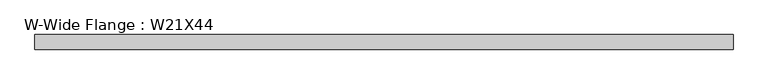
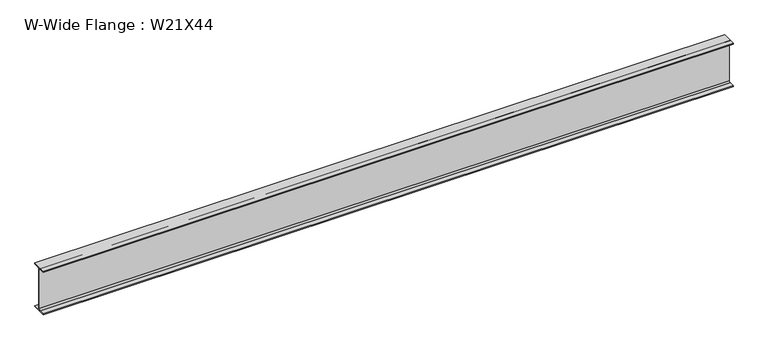
"""IFC4 building model written with IfcOpenShell, lengths in millimetres: beam geometry, W-Wide Flange : W21X44."""

from ifc_helpers import new_model, si_unit, point, frame, frame_2d, origin, place, context, project, spatial, polyline, circle_curve, trimmed, segment, composite_curve, outline, extrude, source, transform, mapped, element, save


def w_wide_flange_w21x44_a0252540(model_context):
    return source(origin(), model_context, "Body", "SweptSolid", [
        extrude(outline(composite_curve([segment(polyline([(82.55, -251.46), (82.55, -262.89), (-82.55, -262.89), (-82.55, -251.46), (-21.59, -251.46)]), True, "CONTINUOUS"), segment(trimmed(circle_curve(frame_2d((-21.59, -234.315)), 17.145), [point((-21.59, -251.46))], [point((-4.445, -234.315))], True, "CARTESIAN"), True, "CONTINUOUS"), segment(polyline([(-4.445, -234.315), (-4.445, 234.315)]), True, "CONTINUOUS"), segment(trimmed(circle_curve(frame_2d((-21.59, 234.315)), 17.145), [point((-4.445, 234.315))], [point((-21.59, 251.46))], True, "CARTESIAN"), True, "CONTINUOUS"), segment(polyline([(-21.59, 251.46), (-82.55, 251.46), (-82.55, 262.89), (82.55, 262.89), (82.55, 251.46), (21.59, 251.46)]), True, "CONTINUOUS"), segment(trimmed(circle_curve(frame_2d((21.59, 234.315)), 17.145), [point((21.59, 251.46))], [point((4.445, 234.315))], True, "CARTESIAN"), True, "CONTINUOUS"), segment(polyline([(4.445, 234.315), (4.445, -234.315)]), True, "CONTINUOUS"), segment(trimmed(circle_curve(frame_2d((21.59, -234.315)), 17.145), [point((4.445, -234.315))], [point((21.59, -251.46))], True, "CARTESIAN"), True, "CONTINUOUS"), segment(polyline([(21.59, -251.46), (82.55, -251.46)]), True, "CONTINUOUS")], self_intersect=False)), frame((-3902.7719693, 0.0, 0.0), z_axis=(1.0, 0.0, 0.0), x_axis=(0.0, 1.0, 0.0)), (0.0, 0.0, 1.0), 7866.2461832),
    ])


if __name__ == "__main__":
    model = new_model("IFC4")
    model_context = context("Model", 3, world=origin())
    ifc_project = project(units=[si_unit("LENGTHUNIT", "METRE", prefix="MILLI")], contexts=[model_context])
    site = spatial("IfcSite", under=ifc_project)
    building = spatial("IfcBuilding", under=site)
    placement = place(None, origin())
    w_wide_flange_w21x44_shape = w_wide_flange_w21x44_a0252540(model_context)
    element("IfcBeam", 1, ObjectType="W-Wide Flange : W21X44", at=placement, inside=building, context=model_context, shape_type="MappedRepresentation", body=[
        mapped(w_wide_flange_w21x44_shape, transform((0.0, 0.0, 0.0), x_axis=(1.0, 0.0, 0.0), y_axis=(0.0, 1.0, 0.0), z_axis=(0.0, 0.0, 1.0))),
    ])
    save(model, "model.ifc")

# Revit data of these elements
# Type "W-Wide Flange : W21X44"
#   Assembly Code = "B10"
#   W = 44
#   Length [instance default] = 1524 mm
#   bf = 165.1 mm
#   d = 525.78 mm
#   k = 28.575 mm
#   k2 = 17.145 mm
#   tf = 11.43 mm
#   tw = 8.89 mm
#   A = 0.00838708 m²
#   Structural Material [instance default] = Steel ASTM A992
# Element 1 (IfcBeam, "W-Wide Flange : W21X44")
#   Structural Material = Aluminum, Anodized Red
#   Materials on its faces: "Aluminum, Anodized Red"
# Materials
#   "Steel ASTM A992": class "Metal", colour RGB 128 0 0, transparency 0, Description = "Structural steel 50ksi", Cost = 0
#   "Aluminum, Anodized Red": class "Metal", colour RGB 120 120 120, transparency 0, Description = "Anodized aluminum, red", Cost = 0
